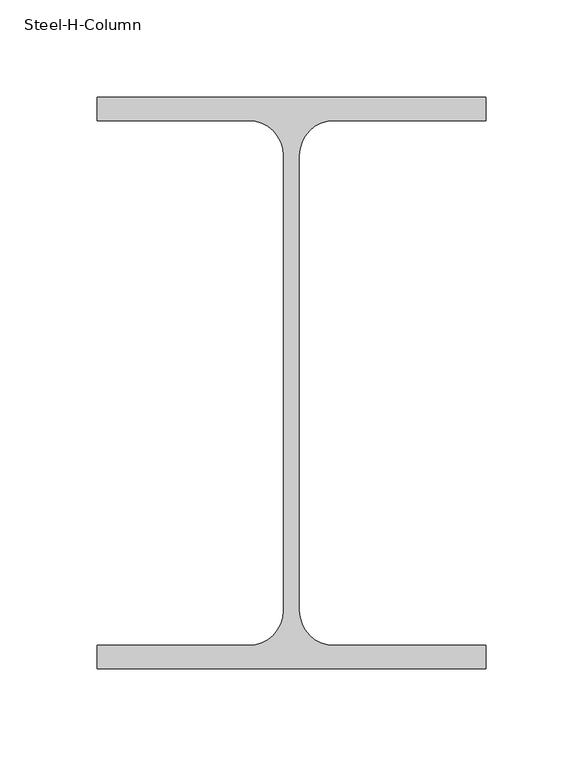
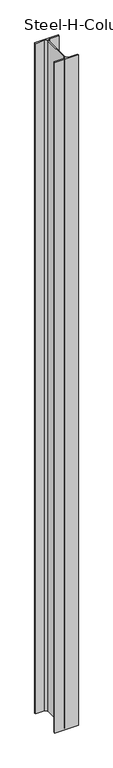
"""IFC4 building model written with IfcOpenShell, lengths in millimetres: column geometry, Steel-H-Column : CL121_H-294×200x8x12."""

from ifc_helpers import new_model, si_unit, point, frame, frame_2d, origin, place, context, project, spatial, polyline, circle_curve, trimmed, segment, composite_curve, outline, extrude, source, transform, mapped, element, save


def steel_h_column_4eecba39(model_context):
    return source(origin(), model_context, "Body", "SweptSolid", [
        extrude(outline(composite_curve([segment(polyline([(100.0, 147.0), (100.0, 135.0), (22.0, 135.0)]), True, "CONTINUOUS"), segment(trimmed(circle_curve(frame_2d((22.0, 117.0)), 18.0), [point((22.0, 135.0))], [point((4.0, 117.0))], True, "CARTESIAN"), True, "CONTINUOUS"), segment(polyline([(4.0, 117.0), (4.0, -117.0)]), True, "CONTINUOUS"), segment(trimmed(circle_curve(frame_2d((22.0, -117.0)), 18.0), [point((4.0, -117.0))], [point((22.0, -135.0))], True, "CARTESIAN"), True, "CONTINUOUS"), segment(polyline([(22.0, -135.0), (100.0, -135.0), (100.0, -147.0), (-100.0, -147.0), (-100.0, -135.0), (-22.0, -135.0)]), True, "CONTINUOUS"), segment(trimmed(circle_curve(frame_2d((-22.0, -117.0)), 18.0), [point((-22.0, -135.0))], [point((-4.0, -117.0))], True, "CARTESIAN"), True, "CONTINUOUS"), segment(polyline([(-4.0, -117.0), (-4.0, 117.0)]), True, "CONTINUOUS"), segment(trimmed(circle_curve(frame_2d((-22.0, 117.0)), 18.0), [point((-4.0, 117.0))], [point((-22.0, 135.0))], True, "CARTESIAN"), True, "CONTINUOUS"), segment(polyline([(-22.0, 135.0), (-100.0, 135.0), (-100.0, 147.0), (100.0, 147.0)]), True, "CONTINUOUS")], self_intersect=False)), frame((0.0, 0.0, 200.0), z_axis=(0.0, 0.0, 1.0), x_axis=(1.0, 0.0, 0.0)), (0.0, 0.0, 1.0), 6000.0),
    ])


if __name__ == "__main__":
    model = new_model("IFC4")
    model_context = context("Model", 3, world=origin())
    ifc_project = project(units=[si_unit("LENGTHUNIT", "METRE", prefix="MILLI")], contexts=[model_context])
    site = spatial("IfcSite", under=ifc_project)
    building = spatial("IfcBuilding", under=site)
    placement = place(None, origin())
    steel_h_column_shape = steel_h_column_4eecba39(model_context)
    element("IfcColumn", 1, ObjectType="Steel-H-Column : CL121_H-294×200x8x12", at=placement, inside=building, context=model_context, shape_type="MappedRepresentation", body=[
        mapped(steel_h_column_shape, transform((0.0, 0.0, 0.0), x_axis=(1.0, 0.0, 0.0), y_axis=(0.0, 1.0, 0.0), z_axis=(0.0, 0.0, 1.0))),
    ])
    save(model, "model.ifc")

# Revit data of these elements
# Type "Steel-H-Column : CL121_H-294×200x8x12"
#   Surface Area = 0.00 m²/m
#   Section Area = 72.38 cm²
#   Mass per Unit Length = 56.80 kg/m
#   B = 200 mm
#   H = 294 mm
#   r = 18 mm
#   tw = 8 mm
#   tf = 12 mm
#   hec_material4 [instance default] = none
#   hec_material2 [instance default] = none
#   hec_material1 [instance default] = none
#   hec_material3 [instance default] = none
#   Structural Material [instance default] = Steel, 45-345
#   Assembly Code = ""
# Element 1 (IfcColumn, "Steel-H-Column : CL121_H-294×200x8x12")
#   hec_material1 = S03AA028-00001_Main Steel Structure Erection Work_Shelter/Building_Medium Steel
#   hec_material3 = F01AC000-00002_Building/Shelter Fire Proofing Work_Intumescent Coating Type_1 hr. rating (UL 1709))
#   Structural Material = S01AA002-00001_Main Steel Structure Fabrication Work_Shelter/Building_Medium Steel - Standard
#   Materials on its faces: "S01AA002-00001_Main Steel Structure Fabrication Work_Shelter/Building_Medium Steel - Standard"
# Materials
#   "Steel, 45-345": class "Metal", colour RGB 189 187 185, transparency 0, Description = "Steel 345 MPa", Cost = 0
#   "S01AA002-00001_Main Steel Structure Fabrication Work_Shelter/Building_Medium Steel - Standard": class "Metal", colour RGB 120 120 120, transparency 0, Comments = "(90KG/M>Weight≥30KG/M)", Description = "Structural steel 50ksi", W00) Work Master Code = "S01AA002-0001", W01) Work Master_Lv1 = "Main Steel Structure Fabrication Work", W02) Work Master_Lv2 = "Shelter/Building", W03) Work Master_Spec.1 = "Medium Steel - Standard (90KG/M>Weight≥30KG/M)", Cost = 0
#   "S03AA028-00001_Main Steel Structure Erection Work_Shelter/Building_Medium Steel": class "Metal", colour RGB 120 120 120, transparency 0, Comments = "(90KG/M>Weight≥30KG/M)", Description = "Structural steel 50ksi", W00) Work Master Code = "S03AA028-0001", W01) Work Master_Lv1 = "Main Steel Structure Erection Work", W02) Work Master_Lv2 = "Shelter/Building", W03) Work Master_Spec.1 = "Medium Steel (90KG/M>Weight≥30KG/M)", Cost = 0
#   "F01AC000-00002_Building/Shelter Fire Proofing Work_Intumescent Coating Type_1 hr. rating (UL 1709))": class "Metal", colour RGB 255 128 128, transparency 0, Description = "Paint finished steel", W00) Work Master Code = "F01AC000-00002", W01) Work Master_Lv1 = "Building/Shelter Fire Proofing Work", W02) Work Master_Lv2 = "Intumescent Coating Type", W03) Work Master_Spec.1 = "1 hr. rating (UL 1709)", Cost = 0
